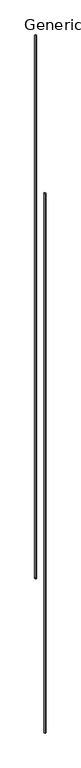
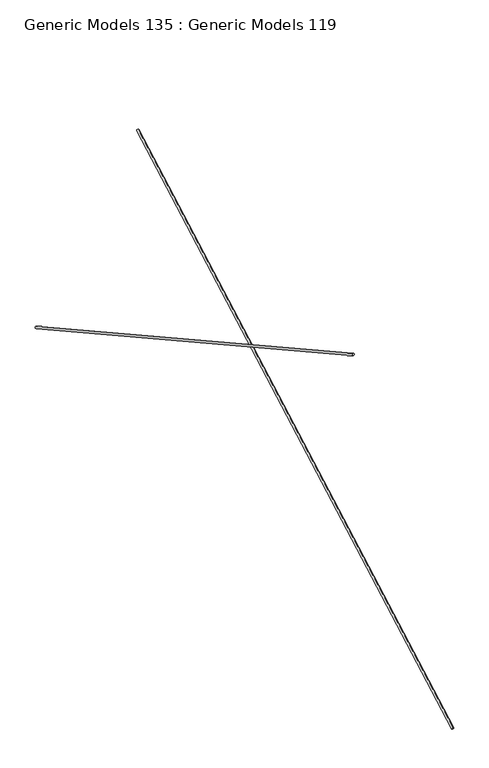
"""IFC4 building model written with IfcOpenShell, lengths in millimetres: proxy geometry, Generic Models 135 : Generic Models 119."""

from ifc_helpers import new_model, si_unit, point, frame, origin, place, context, project, spatial, circle_curve, trimmed, source, transform, mapped, element, save
from ifc_brep_helpers import plane_surface, extruded_surface, advanced_brep


def generic_models_135_generic_models_119_89514f48(model_context):
    return source(origin(), model_context, "Body", "AdvancedBrep", [
        advanced_brep(
        [(32003.9965778, 30873.515427, 269227.0044335), (32003.9965778, 30879.6725092, 269215.8967632), (32002.4450787, 34205.8165112, 271074.1290867), (32002.4450787, 34211.9735934, 271063.0214164)],
        [
            (0, 1, circle_curve(frame((32003.9965778, 30876.5939681, 269221.4505984), z_axis=(0.0, -0.8746197071393959, -0.4848096202463367), x_axis=(0.0, 0.4848096202463367, -0.8746197071393959)), 6.35)),
            (1, 0, circle_curve(frame((32003.9965778, 30876.5939681, 269221.4505984), z_axis=(0.0, -0.8746197071393959, -0.4848096202463367), x_axis=(0.0, 0.4848096202463367, -0.8746197071393959)), 6.35)),
            (2, 3, circle_curve(frame((32002.4450787, 34208.8950523, 271068.5752515), z_axis=(0.0, 0.8746197071393959, 0.4848096202463367), x_axis=(0.0, 0.4848096202463367, -0.8746197071393959)), 6.35)),
            (3, 2, circle_curve(frame((32002.4450787, 34208.8950523, 271068.5752515), z_axis=(0.0, 0.8746197071393959, 0.4848096202463367), x_axis=(0.0, 0.4848096202463367, -0.8746197071393959)), 6.35)),
            (3, 1),
            (0, 2),
        ],
        [
            plane_surface(frame((32003.9965778, 30876.5939681, 269221.4505984), z_axis=(0.0, -0.874619707139396, -0.4848096202463368), x_axis=(-1.0, 0.0, 0.0))),
            plane_surface(frame((32002.4450787, 34208.8950523, 271068.5752515), z_axis=(0.0, 0.874619707139396, 0.4848096202463368), x_axis=(-1.0, 0.0, 0.0))),
            extruded_surface(trimmed(circle_curve(frame((32002.4450787, 34208.8950523, 271068.5752515), z_axis=(0.0, -0.8746197071393959, -0.4848096202463367), x_axis=(0.0, 0.4848096202463367, -0.8746197071393959)), 6.35), [point((32002.4450787, 34205.8165112, 271074.1290867))], [point((32002.4450787, 34211.9735934, 271063.0214164))], True, "CARTESIAN"), (1.55149910000182, -3332.3010842000003, -1847.1246530999779), 3810.0003158792083),
            extruded_surface(trimmed(circle_curve(frame((32002.4450787, 34208.8950523, 271068.5752515), z_axis=(0.0, -0.8746197071393959, -0.4848096202463367), x_axis=(0.0, 0.4848096202463367, -0.8746197071393959)), 6.35), [point((32002.4450787, 34211.9735934, 271063.0214164))], [point((32002.4450787, 34205.8165112, 271074.1290867))], True, "CARTESIAN"), (1.55149910000182, -3332.3010842000003, -1847.1246530999779), 3810.0003158792083),
        ],
        [
            (0, [[1, 2]]),
            (1, [[3, 4]]),
            (2, [[-4, 5, -1, 6]]),
            (3, [[-3, -6, -2, -5]]),
        ],
    ),
        advanced_brep(
        [(31945.3483901, 35181.33255, 269215.8967632), (31945.3483901, 35187.4896321, 269227.0044335), (31945.2937775, 31826.8161252, 271075.3355807), (31945.2937775, 31832.9732074, 271086.443251)],
        [
            (0, 1, circle_curve(frame((31945.3483901, 35184.4110911, 269221.4505984), z_axis=(0.0, 0.874619707139394, -0.48480962024634044), x_axis=(0.0, 0.48480962024634044, 0.874619707139394)), 6.35)),
            (1, 0, circle_curve(frame((31945.3483901, 35184.4110911, 269221.4505984), z_axis=(0.0, 0.874619707139394, -0.48480962024634044), x_axis=(0.0, 0.48480962024634044, 0.874619707139394)), 6.35)),
            (2, 3, circle_curve(frame((31945.2937775, 31829.8946663, 271080.8894159), z_axis=(0.0, -0.874619707139394, 0.48480962024634044), x_axis=(0.0, 0.48480962024634044, 0.874619707139394)), 6.35)),
            (3, 2, circle_curve(frame((31945.2937775, 31829.8946663, 271080.8894159), z_axis=(0.0, -0.874619707139394, 0.48480962024634044), x_axis=(0.0, 0.48480962024634044, 0.874619707139394)), 6.35)),
            (3, 1),
            (0, 2),
        ],
        [
            plane_surface(frame((31945.3483901, 35184.4110911, 269221.4505984), z_axis=(0.0, 0.874619707139394, -0.48480962024634044), x_axis=(-1.0, 0.0, 0.0))),
            plane_surface(frame((31945.2937775, 31829.8946663, 271080.8894159), z_axis=(0.0, -0.874619707139394, 0.48480962024634044), x_axis=(-1.0, 0.0, 0.0))),
            extruded_surface(trimmed(circle_curve(frame((31945.2937775, 31829.8946663, 271080.8894159), z_axis=(0.0, 0.874619707139394, -0.48480962024634044), x_axis=(0.0, 0.48480962024634044, 0.874619707139394)), 6.35), [point((31945.2937775, 31826.8161252, 271075.3355807))], [point((31945.2937775, 31832.9732074, 271086.443251))], True, "CARTESIAN"), (0.05461260000083712, 3354.5164248000037, -1859.4388174999622), 3835.400000425144),
            extruded_surface(trimmed(circle_curve(frame((31945.2937775, 31829.8946663, 271080.8894159), z_axis=(0.0, 0.874619707139394, -0.48480962024634044), x_axis=(0.0, 0.48480962024634044, 0.874619707139394)), 6.35), [point((31945.2937775, 31832.9732074, 271086.443251))], [point((31945.2937775, 31826.8161252, 271075.3355807))], True, "CARTESIAN"), (0.05461260000083712, 3354.5164248000037, -1859.4388174999622), 3835.400000425144),
        ],
        [
            (0, [[1, 2]]),
            (1, [[3, 4]]),
            (2, [[-4, 5, -1, 6]]),
            (3, [[-3, -6, -2, -5]]),
        ],
    ),
    ])


if __name__ == "__main__":
    model = new_model("IFC4")
    model_context = context("Model", 3, world=origin())
    ifc_project = project(units=[si_unit("LENGTHUNIT", "METRE", prefix="MILLI")], contexts=[model_context])
    site = spatial("IfcSite", under=ifc_project)
    building = spatial("IfcBuilding", under=site)
    placement = place(None, origin())
    generic_models_135_generic_models_119_shape = generic_models_135_generic_models_119_89514f48(model_context)
    element("IfcBuildingElementProxy", 1, Name="Generic Models 135 : Generic Models 119", ObjectType="Generic Models 135 : Generic Models 119", at=placement, inside=building, context=model_context, shape_type="MappedRepresentation", body=[
        mapped(generic_models_135_generic_models_119_shape, transform((0.0, 0.0, 0.0), x_axis=(1.0, 0.0, 0.0), y_axis=(0.0, 1.0, 0.0), z_axis=(0.0, 0.0, 1.0))),
    ])
    save(model, "model.ifc")

# Revit data of these elements
# Element 1 (IfcBuildingElementProxy, "Generic Models 135 : Generic Models 119")
#   Materials on its faces: "1/2\" DIA. ROD"
# Materials
#   "1/2\" DIA. ROD": class "Metal", colour RGB 199 199 199, transparency 0, Description = "Carbon steel", Cost = 0
